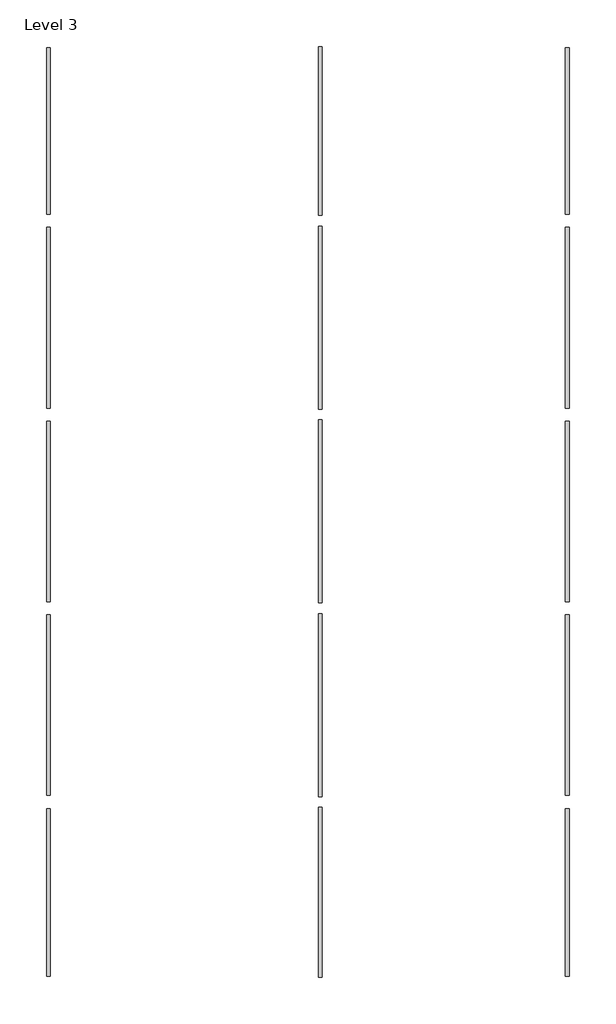
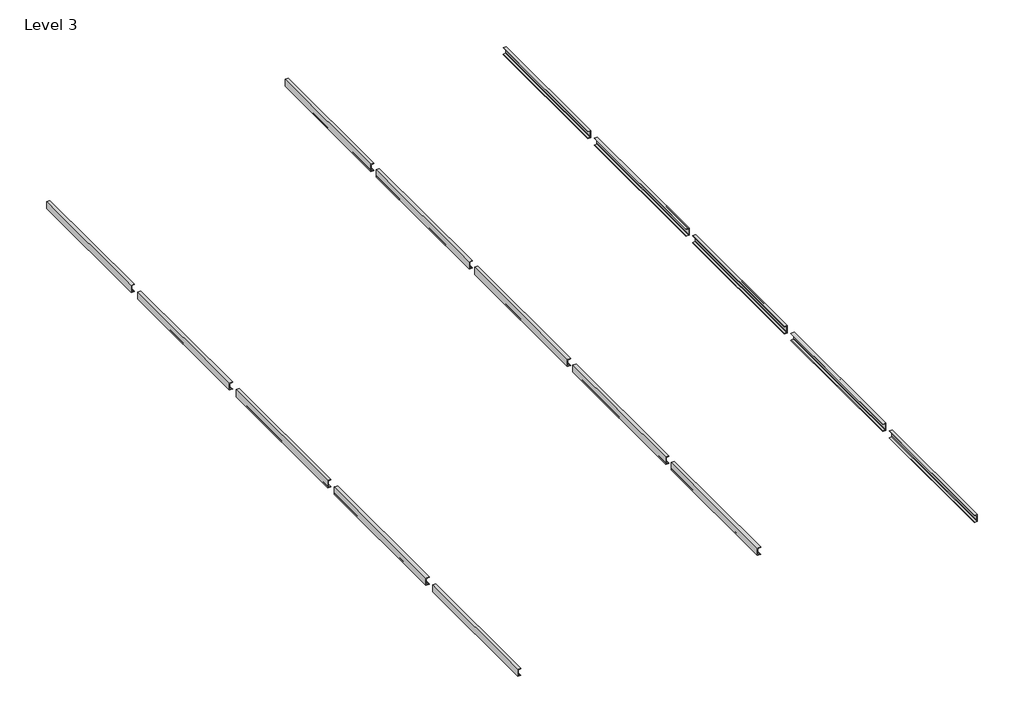
# One storey: 15 beams.
"""IFC4 building model written with IfcOpenShell, lengths in millimetres."""

import ifcopenshell
import ifcopenshell.guid

model = None  # the IFC model being written
_history = None  # IfcOwnerHistory: only IFC2X3 demands one
_inside = {}  # id of a spatial element -> (the spatial element, [elements in it])
_under = {}  # id of a project, library or spatial element -> (it, [spatial elements below it])
_declared = {}  # id of a project -> (the project, [libraries it declares])
_typed = {}  # id of a type object -> (the type object, [elements of that type])
_made_of = {}  # id of a material, layer set ... -> (it, [elements and type objects made of it])


def new_model(schema):
    """Start an empty IFC model of exactly this schema.

    Asked for "IFC4X3", IfcOpenShell would pick the latest addendum, in which some entities
    have other attributes; the version numbers below select the first issue.
    IFC2X3 requires an IfcOwnerHistory on every rooted entity: one is made here for all.
    """
    global model, _history
    if schema == "IFC4X3":
        model = ifcopenshell.file(schema_version=(4, 3, 0, 0))
    else:
        model = ifcopenshell.file(schema=schema)
    _inside.clear()
    _under.clear()
    _declared.clear()
    _typed.clear()
    _made_of.clear()
    _history = None
    if model.schema == "IFC2X3":
        org = make("IfcOrganization", Name="unknown")
        user = make(
            "IfcPersonAndOrganization",
            ThePerson=make("IfcPerson", FamilyName="unknown"),
            TheOrganization=org,
        )
        app = make(
            "IfcApplication",
            ApplicationDeveloper=org,
            Version="unknown",
            ApplicationFullName="unknown",
            ApplicationIdentifier="unknown",
        )
        _history = make(
            "IfcOwnerHistory",
            OwningUser=user,
            OwningApplication=app,
            ChangeAction="ADDED",
            CreationDate=0,
        )
    return model


def make(cls, **values):
    """One entity of the class cls with the attributes given. An attribute that is None is left unset."""
    return model.create_entity(
        cls, **{name: value for name, value in values.items() if value is not None}
    )


def rooted(cls, **values):
    """An entity with a GlobalId (a new one), such as an element, a storey or a relation."""
    return make(cls, GlobalId=ifcopenshell.guid.new(), OwnerHistory=_history, **values)


def si_unit(unit_type, name, prefix=None):
    """IfcSIUnit, for example si_unit("LENGTHUNIT", "METRE", prefix="MILLI")."""
    return make("IfcSIUnit", UnitType=unit_type, Prefix=prefix, Name=name)


def assignment(units):
    """IfcUnitAssignment: the units of a project."""
    return None if units is None else make("IfcUnitAssignment", Units=units)


def point(xyz):
    """IfcCartesianPoint."""
    return None if xyz is None else make("IfcCartesianPoint", Coordinates=xyz)


def direction(xyz):
    """IfcDirection."""
    return None if xyz is None else make("IfcDirection", DirectionRatios=xyz)


def frame(location, z_axis=None, x_axis=None):
    """IfcAxis2Placement3D, a coordinate frame: its origin and axes. An axis left out is left unset."""
    return make(
        "IfcAxis2Placement3D",
        Location=point(location),
        Axis=direction(z_axis),
        RefDirection=direction(x_axis),
    )


def frame_2d(location, x_axis=None):
    """IfcAxis2Placement2D, a coordinate frame in the plane: its origin and x axis."""
    return make(
        "IfcAxis2Placement2D", Location=point(location), RefDirection=direction(x_axis)
    )


def origin():
    """The frame at (0, 0, 0) with its axes left unset."""
    return frame((0.0, 0.0, 0.0))


def place(relative_to, where):
    """IfcLocalPlacement: puts the frame where relative to a parent placement (None: the world)."""
    return make(
        "IfcLocalPlacement", PlacementRelTo=relative_to, RelativePlacement=where
    )


def context(
    kind, dimensions, precision=None, world=None, true_north=None, identifier=None
):
    """IfcGeometricRepresentationContext, for example the 3D "Model" context."""
    return make(
        "IfcGeometricRepresentationContext",
        ContextIdentifier=identifier,
        ContextType=kind,
        CoordinateSpaceDimension=dimensions,
        Precision=precision,
        WorldCoordinateSystem=world,
        TrueNorth=true_north,
    )


def project(units=None, contexts=None):
    """IfcProject with its units and contexts."""
    return rooted(
        "IfcProject",
        Name="project",
        RepresentationContexts=contexts,
        UnitsInContext=assignment(units),
    )


def spatial(cls, under=None, at=None, **own):
    """A site, building, storey or space (cls), placed at a placement, below another one or the project."""
    s = rooted(cls, ObjectPlacement=at, **own)
    if under is not None:
        _under.setdefault(under.id(), (under, []))[1].append(s)
    return s


def polyline(points):
    """IfcPolyline through the points."""
    return make("IfcPolyline", Points=[point(p) for p in points])


def circle_curve(where, radius):
    """IfcCircle in the frame where."""
    return make("IfcCircle", Position=where, Radius=radius)


def trimmed(basis, trim1, trim2, sense, master):
    """IfcTrimmedCurve: the piece of a basis curve between two trims."""
    return make(
        "IfcTrimmedCurve",
        BasisCurve=basis,
        Trim1=trim1,
        Trim2=trim2,
        SenseAgreement=sense,
        MasterRepresentation=master,
    )


def segment(curve, same_sense, transition):
    """IfcCompositeCurveSegment."""
    return make(
        "IfcCompositeCurveSegment",
        Transition=transition,
        SameSense=same_sense,
        ParentCurve=curve,
    )


def composite_curve(segments, self_intersect=None):
    """IfcCompositeCurve: segments joined end to end."""
    return make("IfcCompositeCurve", Segments=segments, SelfIntersect=self_intersect)


def outline(outer, holes=None, kind="AREA"):
    """IfcArbitraryClosedProfileDef: a profile drawn as a closed curve; with holes, ...WithVoids."""
    if holes is None:
        return make("IfcArbitraryClosedProfileDef", ProfileType=kind, OuterCurve=outer)
    return make(
        "IfcArbitraryProfileDefWithVoids",
        ProfileType=kind,
        OuterCurve=outer,
        InnerCurves=holes,
    )


def extrude(swept, where, along, depth):
    """IfcExtrudedAreaSolid: the profile swept, set in the frame where, extruded along a direction by depth."""
    return make(
        "IfcExtrudedAreaSolid",
        SweptArea=swept,
        Position=where,
        ExtrudedDirection=direction(along),
        Depth=depth,
    )


def shape(context_of_items, identifier, shape_type, items):
    """IfcShapeRepresentation: the items that make up one representation, for example the "Body"."""
    return make(
        "IfcShapeRepresentation",
        ContextOfItems=context_of_items,
        RepresentationIdentifier=identifier,
        RepresentationType=shape_type,
        Items=items,
    )


def source(mapping_origin, context_of_items, identifier, shape_type, items):
    """IfcRepresentationMap: a shape defined once, which mapped items show again and again."""
    return make(
        "IfcRepresentationMap",
        MappingOrigin=mapping_origin,
        MappedRepresentation=shape(context_of_items, identifier, shape_type, items),
    )


def transform(
    local_origin,
    x_axis=None,
    y_axis=None,
    z_axis=None,
    scale=None,
    scale2=None,
    scale3=None,
    uniform=True,
):
    """IfcCartesianTransformationOperator3D, or its non-uniform kind. x_axis, y_axis, z_axis: its Axis1, 2, 3."""
    if uniform:
        return make(
            "IfcCartesianTransformationOperator3D",
            Axis1=direction(x_axis),
            Axis2=direction(y_axis),
            LocalOrigin=point(local_origin),
            Scale=scale,
            Axis3=direction(z_axis),
        )
    return make(
        "IfcCartesianTransformationOperator3DnonUniform",
        Axis1=direction(x_axis),
        Axis2=direction(y_axis),
        LocalOrigin=point(local_origin),
        Scale=scale,
        Axis3=direction(z_axis),
        Scale2=scale2,
        Scale3=scale3,
    )


def mapped(mapping_source, mapping_target):
    """IfcMappedItem: shows the shape of a source again, moved by a transform."""
    return make(
        "IfcMappedItem", MappingSource=mapping_source, MappingTarget=mapping_target
    )


def made_of(thing, what):
    """Note that an element or type object is made of a material, layer set ...; save() writes the relation."""
    if what is not None:
        _made_of.setdefault(what.id(), (what, []))[1].append(thing)
    return thing


def element(
    cls,
    number,
    at=None,
    inside=None,
    cuts=None,
    type_object=None,
    material=None,
    context=None,
    identifier="Body",
    shape_type=None,
    held_by="IfcProductDefinitionShape",
    body=None,
    shapes=None,
    **own,
):
    """One element of the class cls, such as IfcWall. Its Tag is "e" and its number.

    at: its placement. inside: the storey or other place that contains it. cuts: it is an
    opening in that element (IfcRelVoidsElement). A single representation is given by context,
    identifier, shape_type and body (its items); several are given by shapes. held_by: the class
    of the entity that holds the representations. save() writes the other relations.
    """
    e = rooted(cls, Tag="e%d" % number, ObjectPlacement=at, **own)
    if body is not None:
        shapes = [shape(context, identifier, shape_type, body)]
    if shapes is not None:
        e.Representation = make(held_by, Representations=shapes)
    if inside is not None:
        _inside.setdefault(inside.id(), (inside, []))[1].append(e)
    if cuts is not None:
        rooted(
            "IfcRelVoidsElement", RelatingBuildingElement=cuts, RelatedOpeningElement=e
        )
    if type_object is not None:
        _typed.setdefault(type_object.id(), (type_object, []))[1].append(e)
    return made_of(e, material)


def aggregate(whole, parts):
    """IfcRelAggregates: a whole, such as a stair, and the parts it consists of."""
    return rooted("IfcRelAggregates", RelatingObject=whole, RelatedObjects=parts)


def save(model, path):
    """Write the relations noted so far, then the file.

    IfcRelAggregates (storeys below a building ...), IfcRelContainedInSpatialStructure (elements
    in a storey), IfcRelDefinesByType, IfcRelAssociatesMaterial and IfcRelDeclares: one each for
    every whole, place, type object, material and project.
    """
    for whole, parts in _under.values():
        aggregate(whole, parts)
    for where, things in _inside.values():
        rooted(
            "IfcRelContainedInSpatialStructure",
            RelatedElements=things,
            RelatingStructure=where,
        )
    for kind, things in _typed.values():
        rooted("IfcRelDefinesByType", RelatedObjects=things, RelatingType=kind)
    for what, things in _made_of.values():
        rooted("IfcRelAssociatesMaterial", RelatedObjects=things, RelatingMaterial=what)
    for by, libraries in _declared.values():
        rooted("IfcRelDeclares", RelatingContext=by, RelatedDefinitions=libraries)
    model.write(path)


def c_shapes_c4x6_25_9ff4ea91(model_context):
    return source(origin(), model_context, "Body", "SweptSolid", [
        extrude(outline(composite_curve([segment(polyline([(11.049, 50.8), (11.049, -50.8), (-30.861, -50.8), (-30.861, -49.7865772)]), True, "CONTINUOUS"), segment(trimmed(circle_curve(frame_2d((-27.4066, -49.7865772)), 3.4544), [point((-30.861, -49.7865772))], [point((-27.9743618, -46.379155))], False, "CARTESIAN"), True, "CONTINUOUS"), segment(polyline([(-27.9743618, -46.379155), (-0.9980765, -41.8842311)]), True, "CONTINUOUS"), segment(trimmed(circle_curve(frame_2d((-2.1336, -35.0693868)), 6.9088), [point((-0.9980765, -41.8842311))], [point((4.7752, -35.0693868))], True, "CARTESIAN"), True, "CONTINUOUS"), segment(polyline([(4.7752, -35.0693868), (4.7752, 35.0693868)]), True, "CONTINUOUS"), segment(trimmed(circle_curve(frame_2d((-2.1336, 35.0693868)), 6.9088), [point((4.7752, 35.0693868))], [point((-0.9980765, 41.8842311))], True, "CARTESIAN"), True, "CONTINUOUS"), segment(polyline([(-0.9980765, 41.8842311), (-27.9743618, 46.379155)]), True, "CONTINUOUS"), segment(trimmed(circle_curve(frame_2d((-27.4066, 49.7865772)), 3.4544), [point((-27.9743618, 46.379155))], [point((-30.861, 49.7865772))], False, "CARTESIAN"), True, "CONTINUOUS"), segment(polyline([(-30.861, 49.7865772), (-30.861, 50.8), (11.049, 50.8)]), True, "CONTINUOUS")], self_intersect=False)), frame((-1049.3744237, 0.0, 0.0), z_axis=(1.0, 0.0, 0.0), x_axis=(0.0, 1.0, 0.0)), (0.0, 0.0, 1.0), 2098.7488474),
    ])


def c_shapes_c4x6_25_a736a65e(model_context):
    return source(origin(), model_context, "Body", "SweptSolid", [
        extrude(outline(composite_curve([segment(polyline([(11.049, 50.8), (11.049, -50.8), (-30.861, -50.8), (-30.861, -49.7865772)]), True, "CONTINUOUS"), segment(trimmed(circle_curve(frame_2d((-27.4066, -49.7865772)), 3.4544), [point((-30.861, -49.7865772))], [point((-27.9743618, -46.379155))], False, "CARTESIAN"), True, "CONTINUOUS"), segment(polyline([(-27.9743618, -46.379155), (-0.9980765, -41.8842311)]), True, "CONTINUOUS"), segment(trimmed(circle_curve(frame_2d((-2.1336, -35.0693868)), 6.9088), [point((-0.9980765, -41.8842311))], [point((4.7752, -35.0693868))], True, "CARTESIAN"), True, "CONTINUOUS"), segment(polyline([(4.7752, -35.0693868), (4.7752, 35.0693868)]), True, "CONTINUOUS"), segment(trimmed(circle_curve(frame_2d((-2.1336, 35.0693868)), 6.9088), [point((4.7752, 35.0693868))], [point((-0.9980765, 41.8842311))], True, "CARTESIAN"), True, "CONTINUOUS"), segment(polyline([(-0.9980765, 41.8842311), (-27.9743618, 46.379155)]), True, "CONTINUOUS"), segment(trimmed(circle_curve(frame_2d((-27.4066, 49.7865772)), 3.4544), [point((-27.9743618, 46.379155))], [point((-30.861, 49.7865772))], False, "CARTESIAN"), True, "CONTINUOUS"), segment(polyline([(-30.861, 49.7865772), (-30.861, 50.8), (11.049, 50.8)]), True, "CONTINUOUS")], self_intersect=False)), frame((-974.344, 0.0, 0.0), z_axis=(1.0, 0.0, 0.0), x_axis=(0.0, 1.0, 0.0)), (0.0, 0.0, 1.0), 1948.688),
    ])


def c_shapes_c4x6_25_c3130f21(model_context):
    return source(origin(), model_context, "Body", "SweptSolid", [
        extrude(outline(composite_curve([segment(polyline([(11.049, 50.8), (11.049, -50.8), (-30.861, -50.8), (-30.861, -49.7865772)]), True, "CONTINUOUS"), segment(trimmed(circle_curve(frame_2d((-27.4066, -49.7865772)), 3.4544), [point((-30.861, -49.7865772))], [point((-27.9743618, -46.379155))], False, "CARTESIAN"), True, "CONTINUOUS"), segment(polyline([(-27.9743618, -46.379155), (-0.9980765, -41.8842311)]), True, "CONTINUOUS"), segment(trimmed(circle_curve(frame_2d((-2.1336, -35.0693868)), 6.9088), [point((-0.9980765, -41.8842311))], [point((4.7752, -35.0693868))], True, "CARTESIAN"), True, "CONTINUOUS"), segment(polyline([(4.7752, -35.0693868), (4.7752, 35.0693868)]), True, "CONTINUOUS"), segment(trimmed(circle_curve(frame_2d((-2.1336, 35.0693868)), 6.9088), [point((4.7752, 35.0693868))], [point((-0.9980765, 41.8842311))], True, "CARTESIAN"), True, "CONTINUOUS"), segment(polyline([(-0.9980765, 41.8842311), (-27.9743618, 46.379155)]), True, "CONTINUOUS"), segment(trimmed(circle_curve(frame_2d((-27.4066, 49.7865772)), 3.4544), [point((-27.9743618, 46.379155))], [point((-30.861, 49.7865772))], False, "CARTESIAN"), True, "CONTINUOUS"), segment(polyline([(-30.861, 49.7865772), (-30.861, 50.8), (11.049, 50.8)]), True, "CONTINUOUS")], self_intersect=False)), frame((-967.994, 0.0, 0.0), z_axis=(1.0, 0.0, 0.0), x_axis=(0.0, 1.0, 0.0)), (0.0, 0.0, 1.0), 1935.988),
    ])


def c_shapes_c4x6_25_2e0b3a68(model_context):
    return source(origin(), model_context, "Body", "SweptSolid", [
        extrude(outline(composite_curve([segment(polyline([(11.049, 50.8), (11.049, -50.8), (-30.861, -50.8), (-30.861, -49.7865772)]), True, "CONTINUOUS"), segment(trimmed(circle_curve(frame_2d((-27.4066, -49.7865772)), 3.4544), [point((-30.861, -49.7865772))], [point((-27.9743618, -46.379155))], False, "CARTESIAN"), True, "CONTINUOUS"), segment(polyline([(-27.9743618, -46.379155), (-0.9980765, -41.8842311)]), True, "CONTINUOUS"), segment(trimmed(circle_curve(frame_2d((-2.1336, -35.0693868)), 6.9088), [point((-0.9980765, -41.8842311))], [point((4.7752, -35.0693868))], True, "CARTESIAN"), True, "CONTINUOUS"), segment(polyline([(4.7752, -35.0693868), (4.7752, 35.0693868)]), True, "CONTINUOUS"), segment(trimmed(circle_curve(frame_2d((-2.1336, 35.0693868)), 6.9088), [point((4.7752, 35.0693868))], [point((-0.9980765, 41.8842311))], True, "CARTESIAN"), True, "CONTINUOUS"), segment(polyline([(-0.9980765, 41.8842311), (-27.9743618, 46.379155)]), True, "CONTINUOUS"), segment(trimmed(circle_curve(frame_2d((-27.4066, 49.7865772)), 3.4544), [point((-27.9743618, 46.379155))], [point((-30.861, 49.7865772))], False, "CARTESIAN"), True, "CONTINUOUS"), segment(polyline([(-30.861, 49.7865772), (-30.861, 50.8), (11.049, 50.8)]), True, "CONTINUOUS")], self_intersect=False)), frame((-988.187, 0.0, 0.0), z_axis=(1.0, 0.0, 0.0), x_axis=(0.0, 1.0, 0.0)), (0.0, 0.0, 1.0), 1976.374),
    ])


def c_shapes_c4x6_25_cfd2a1e4(model_context):
    return source(origin(), model_context, "Body", "SweptSolid", [
        extrude(outline(composite_curve([segment(polyline([(11.049, 50.8), (11.049, -50.8), (-30.861, -50.8), (-30.861, -49.7865772)]), True, "CONTINUOUS"), segment(trimmed(circle_curve(frame_2d((-27.4066, -49.7865772)), 3.4544), [point((-30.861, -49.7865772))], [point((-27.9743618, -46.379155))], False, "CARTESIAN"), True, "CONTINUOUS"), segment(polyline([(-27.9743618, -46.379155), (-0.9980765, -41.8842311)]), True, "CONTINUOUS"), segment(trimmed(circle_curve(frame_2d((-2.1336, -35.0693868)), 6.9088), [point((-0.9980765, -41.8842311))], [point((4.7752, -35.0693868))], True, "CARTESIAN"), True, "CONTINUOUS"), segment(polyline([(4.7752, -35.0693868), (4.7752, 35.0693868)]), True, "CONTINUOUS"), segment(trimmed(circle_curve(frame_2d((-2.1336, 35.0693868)), 6.9088), [point((4.7752, 35.0693868))], [point((-0.9980765, 41.8842311))], True, "CARTESIAN"), True, "CONTINUOUS"), segment(polyline([(-0.9980765, 41.8842311), (-27.9743618, 46.379155)]), True, "CONTINUOUS"), segment(trimmed(circle_curve(frame_2d((-27.4066, 49.7865772)), 3.4544), [point((-27.9743618, 46.379155))], [point((-30.861, 49.7865772))], False, "CARTESIAN"), True, "CONTINUOUS"), segment(polyline([(-30.861, 49.7865772), (-30.861, 50.8), (11.049, 50.8)]), True, "CONTINUOUS")], self_intersect=False)), frame((-1063.2174237, 0.0, 0.0), z_axis=(1.0, 0.0, 0.0), x_axis=(0.0, 1.0, 0.0)), (0.0, 0.0, 1.0), 2126.4348474),
    ])


def c_shapes_c4x6_25_45f65e66(model_context):
    return source(origin(), model_context, "Body", "SweptSolid", [
        extrude(outline(composite_curve([segment(polyline([(11.049, 50.8), (11.049, -50.8), (-30.861, -50.8), (-30.861, -49.7865772)]), True, "CONTINUOUS"), segment(trimmed(circle_curve(frame_2d((-27.4066, -49.7865772)), 3.4544), [point((-30.861, -49.7865772))], [point((-27.9743618, -46.379155))], False, "CARTESIAN"), True, "CONTINUOUS"), segment(polyline([(-27.9743618, -46.379155), (-0.9980765, -41.8842311)]), True, "CONTINUOUS"), segment(trimmed(circle_curve(frame_2d((-2.1336, -35.0693868)), 6.9088), [point((-0.9980765, -41.8842311))], [point((4.7752, -35.0693868))], True, "CARTESIAN"), True, "CONTINUOUS"), segment(polyline([(4.7752, -35.0693868), (4.7752, 35.0693868)]), True, "CONTINUOUS"), segment(trimmed(circle_curve(frame_2d((-2.1336, 35.0693868)), 6.9088), [point((4.7752, 35.0693868))], [point((-0.9980765, 41.8842311))], True, "CARTESIAN"), True, "CONTINUOUS"), segment(polyline([(-0.9980765, 41.8842311), (-27.9743618, 46.379155)]), True, "CONTINUOUS"), segment(trimmed(circle_curve(frame_2d((-27.4066, 49.7865772)), 3.4544), [point((-27.9743618, 46.379155))], [point((-30.861, 49.7865772))], False, "CARTESIAN"), True, "CONTINUOUS"), segment(polyline([(-30.861, 49.7865772), (-30.861, 50.8), (11.049, 50.8)]), True, "CONTINUOUS")], self_intersect=False)), frame((-981.837, 0.0, 0.0), z_axis=(1.0, 0.0, 0.0), x_axis=(0.0, 1.0, 0.0)), (0.0, 0.0, 1.0), 1963.674),
    ])


model = new_model("IFC4")

# Units and contexts
model_context = context("Model", 3, world=origin())
ifc_project = project(units=[si_unit("LENGTHUNIT", "METRE", prefix="MILLI")], contexts=[model_context])

# Site, building, storey
site = spatial("IfcSite", under=ifc_project)
building = spatial("IfcBuilding", under=site)
storey = spatial("IfcBuildingStorey", under=building, Name="Level 3", Elevation=6096.0)

# Beams
placement = place(None, origin())
c_shapes_c4x6_25_shape = c_shapes_c4x6_25_9ff4ea91(model_context)
element("IfcBeam", 1, ObjectType="C Shapes : C4X6.25", at=placement, inside=storey, context=model_context, shape_type="MappedRepresentation", body=[
    mapped(c_shapes_c4x6_25_shape, transform((-156.8401664, 7881.4478769, 5825.1336143), x_axis=(0.0, -1.0, 0.0), y_axis=(1.0, 0.0, 0.0), z_axis=(0.0, 0.0, 1.0))),
])
element("IfcBeam", 2, ObjectType="C Shapes : C4X6.25", at=placement, inside=storey, context=model_context, shape_type="MappedRepresentation", body=[
    mapped(c_shapes_c4x6_25_shape, transform((-156.8401664, 5629.5370295, 5825.1336143), x_axis=(0.0, -1.0, 0.0), y_axis=(1.0, 0.0, 0.0), z_axis=(0.0, 0.0, 1.0))),
])
element("IfcBeam", 3, ObjectType="C Shapes : C4X6.25", at=placement, inside=storey, context=model_context, shape_type="MappedRepresentation", body=[
    mapped(c_shapes_c4x6_25_shape, transform((-156.8401664, 3377.6261821, 5825.1336143), x_axis=(0.0, -1.0, 0.0), y_axis=(1.0, 0.0, 0.0), z_axis=(0.0, 0.0, 1.0))),
])
element("IfcBeam", 4, ObjectType="C Shapes : C4X6.25", at=placement, inside=storey, context=model_context, shape_type="MappedRepresentation", body=[
    mapped(c_shapes_c4x6_25_shape, transform((-6214.7401664, 3377.6261821, 5786.3114063), x_axis=(0.0, 1.0, 0.0), y_axis=(-1.0, 0.0, 0.0), z_axis=(0.0, 0.0, 1.0))),
])
element("IfcBeam", 5, ObjectType="C Shapes : C4X6.25", at=placement, inside=storey, context=model_context, shape_type="MappedRepresentation", body=[
    mapped(c_shapes_c4x6_25_shape, transform((-6214.7401664, 5629.5370295, 5786.3114063), x_axis=(0.0, 1.0, 0.0), y_axis=(-1.0, 0.0, 0.0), z_axis=(0.0, 0.0, 1.0))),
])
element("IfcBeam", 6, ObjectType="C Shapes : C4X6.25", at=placement, inside=storey, context=model_context, shape_type="MappedRepresentation", body=[
    mapped(c_shapes_c4x6_25_shape, transform((-6214.7401664, 7881.4478769, 5786.3114063), x_axis=(0.0, 1.0, 0.0), y_axis=(-1.0, 0.0, 0.0), z_axis=(0.0, 0.0, 1.0))),
])
c_shapes_c4x6_25_2_shape = c_shapes_c4x6_25_a736a65e(model_context)
element("IfcBeam", 7, ObjectType="C Shapes : C4X6.25", at=placement, inside=storey, context=model_context, shape_type="MappedRepresentation", body=[
    mapped(c_shapes_c4x6_25_2_shape, transform((-156.8401664, 1200.7457583, 5825.1336143), x_axis=(0.0, -1.0, 0.0), y_axis=(1.0, 0.0, 0.0), z_axis=(0.0, 0.0, 1.0))),
])
element("IfcBeam", 8, ObjectType="C Shapes : C4X6.25", at=placement, inside=storey, context=model_context, shape_type="MappedRepresentation", body=[
    mapped(c_shapes_c4x6_25_2_shape, transform((-6214.7401664, 1200.7457583, 5786.3114063), x_axis=(0.0, 1.0, 0.0), y_axis=(-1.0, 0.0, 0.0), z_axis=(0.0, 0.0, 1.0))),
])
c_shapes_c4x6_25_3_shape = c_shapes_c4x6_25_c3130f21(model_context)
element("IfcBeam", 9, ObjectType="C Shapes : C4X6.25", at=placement, inside=storey, context=model_context, shape_type="MappedRepresentation", body=[
    mapped(c_shapes_c4x6_25_3_shape, transform((-156.8401664, 10051.9783006, 5825.1336143), x_axis=(0.0, -1.0, 0.0), y_axis=(1.0, 0.0, 0.0), z_axis=(0.0, 0.0, 1.0))),
])
element("IfcBeam", 10, ObjectType="C Shapes : C4X6.25", at=placement, inside=storey, context=model_context, shape_type="MappedRepresentation", body=[
    mapped(c_shapes_c4x6_25_3_shape, transform((-6214.7401664, 10051.9783006, 5786.3114063), x_axis=(0.0, 1.0, 0.0), y_axis=(-1.0, 0.0, 0.0), z_axis=(0.0, 0.0, 1.0))),
])
c_shapes_c4x6_25_4_shape = c_shapes_c4x6_25_2e0b3a68(model_context)
element("IfcBeam", 11, ObjectType="C Shapes : C4X6.25", at=placement, inside=storey, context=model_context, shape_type="MappedRepresentation", body=[
    mapped(c_shapes_c4x6_25_4_shape, transform((-3052.4401664, 1200.7457583, 6381.6839899), x_axis=(0.0, 1.0, 0.0), y_axis=(-1.0, 0.0, 0.0), z_axis=(0.0, 0.0, 1.0))),
])
c_shapes_c4x6_25_5_shape = c_shapes_c4x6_25_cfd2a1e4(model_context)
element("IfcBeam", 12, ObjectType="C Shapes : C4X6.25", at=placement, inside=storey, context=model_context, shape_type="MappedRepresentation", body=[
    mapped(c_shapes_c4x6_25_5_shape, transform((-3052.4401664, 3377.6261821, 6381.6839899), x_axis=(0.0, 1.0, 0.0), y_axis=(-1.0, 0.0, 0.0), z_axis=(0.0, 0.0, 1.0))),
])
element("IfcBeam", 13, ObjectType="C Shapes : C4X6.25", at=placement, inside=storey, context=model_context, shape_type="MappedRepresentation", body=[
    mapped(c_shapes_c4x6_25_5_shape, transform((-3052.4401664, 5629.5370295, 6381.6839899), x_axis=(0.0, 1.0, 0.0), y_axis=(-1.0, 0.0, 0.0), z_axis=(0.0, 0.0, 1.0))),
])
element("IfcBeam", 14, ObjectType="C Shapes : C4X6.25", at=placement, inside=storey, context=model_context, shape_type="MappedRepresentation", body=[
    mapped(c_shapes_c4x6_25_5_shape, transform((-3052.4401664, 7881.4478769, 6381.6839899), x_axis=(0.0, 1.0, 0.0), y_axis=(-1.0, 0.0, 0.0), z_axis=(0.0, 0.0, 1.0))),
])
c_shapes_c4x6_25_6_shape = c_shapes_c4x6_25_45f65e66(model_context)
element("IfcBeam", 15, ObjectType="C Shapes : C4X6.25", at=placement, inside=storey, context=model_context, shape_type="MappedRepresentation", body=[
    mapped(c_shapes_c4x6_25_6_shape, transform((-3052.4401664, 10051.9783006, 6381.6839899), x_axis=(0.0, 1.0, 0.0), y_axis=(-1.0, 0.0, 0.0), z_axis=(0.0, 0.0, 1.0))),
])

save(model, "model.ifc")

# Revit data of these elements
# Type "C Shapes : C4X6.25"
#   Section Name Key = "ChannelsC4X6.25"
#   Assembly Code = "B10"
#   Width = 1.650"
#   Web Thickness = 0.247"
#   Web Fillet = 0.272"
#   Warping Constant = 1.03 in⁶
#   Torsional Moment of Inertia = 0.0487 in⁴
#   Sloped Flange Angle = 9.46°
#   Section Area = 1.77 in²
#   Plastic Modulus weak axis = 0.569 in³
#   Plastic Modulus strong axis = 2.43 in³
#   Nominal Weight = 6.25 lbf/ft
#   Moment of Inertia weak axis = 0.345 in⁴
#   Moment of Inertia strong axis = 4.00 in⁴
#   Height = 4.000"
#   Flange Thickness Location = 0.7015"
#   Flange Thickness = 0.272"
#   Flange Fillet = 0.136"
#   Elastic Modulus weak axis = 0.284 in³
#   Elastic Modulus strong axis = 2.00 in³
#   Centroid Vertical = 2.000"
#   Centroid Horizontal = 0.435"
#   Length [instance default] = 5' - 0"
#   Structural Material [instance default] = Steel ASTM A36
#   Principal Axes Angle = 0
#   Bolt Spacing = 0
# Elements 1, 2, 3, 4, 5, 6, 7, 8, 9, 10, 11, 12, 13, 14, 15 (IfcBeam, "C Shapes : C4X6.25")
#   Structural Material = Steel ASTM A36
#   Phase Created = New Construction
#   Materials on its faces: "Steel ASTM A36"
# Materials
#   "Steel ASTM A36": class "Metal", colour RGB 199 199 199, transparency 0, Description = "Structural steel, ASTM A36 Grade B, mill finish", Cost = 0
